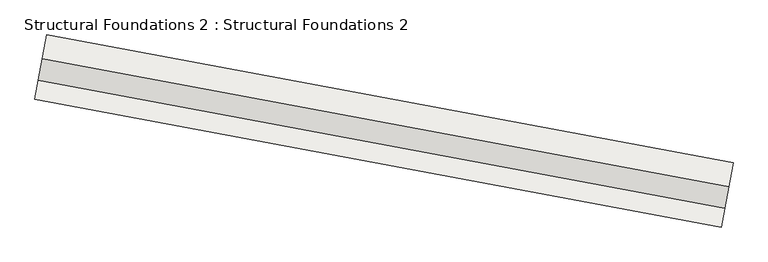
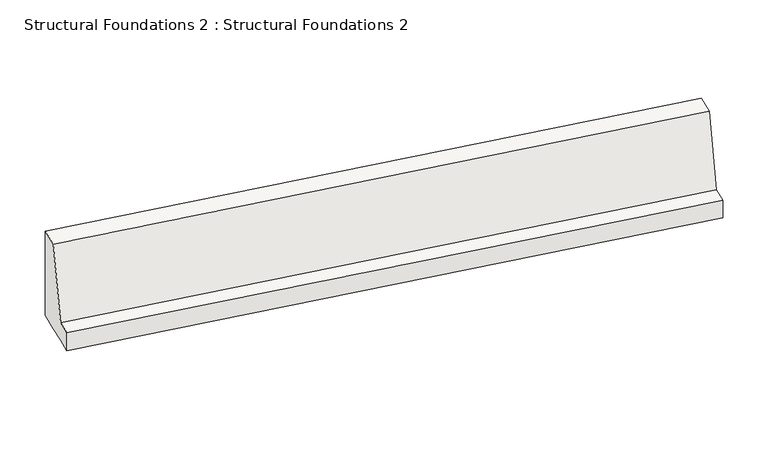
"""IFC4 building model written with IfcOpenShell, lengths in millimetres: slab geometry, Structural Foundations 2 : Structural Foundations 2."""

from ifc_helpers import new_model, si_unit, frame, origin, place, context, project, spatial, polyline, outline, extrude, source, transform, mapped, element, save


def structural_foundations_2_structural_foundations_2_d3b20905(model_context):
    return source(origin(), model_context, "Body", "SweptSolid", [
        extrude(outline(polyline([(0.0, 0.0), (0.0, -1930.4), (-457.2, -1930.4), (-863.6, -406.4), (-1219.2, -406.4), (-1219.2, 0.0), (-863.6, 0.0), (-457.2, 0.0), (0.0, 0.0)])), frame((-47568.5974532, 36188.2727948, 7848.6), z_axis=(-0.9830688624224049, 0.18323649127703542, 0.0), x_axis=(0.18323649127703542, 0.9830688624224049, 0.0)), (0.0, 0.0, 1.0), 13030.2),
    ])


if __name__ == "__main__":
    model = new_model("IFC4")
    model_context = context("Model", 3, world=origin())
    ifc_project = project(units=[si_unit("LENGTHUNIT", "METRE", prefix="MILLI")], contexts=[model_context])
    site = spatial("IfcSite", under=ifc_project)
    building = spatial("IfcBuilding", under=site)
    placement = place(None, origin())
    structural_foundations_2_structural_foundations_2_shape = structural_foundations_2_structural_foundations_2_d3b20905(model_context)
    element("IfcSlab", 1, ObjectType="Structural Foundations 2 : Structural Foundations 2", at=placement, inside=building, context=model_context, shape_type="MappedRepresentation", body=[
        mapped(structural_foundations_2_structural_foundations_2_shape, transform((0.0, 0.0, 0.0), x_axis=(1.0, 0.0, 0.0), y_axis=(0.0, 1.0, 0.0), z_axis=(0.0, 0.0, 1.0))),
    ])
    save(model, "model.ifc")

# Revit data of these elements
# Element 1 (IfcSlab, "Structural Foundations 2 : Structural Foundations 2")
#   Materials on its faces: "16 - Concrete - Cast-in-Place"
# Materials
#   "16 - Concrete - Cast-in-Place": class "Unassigned", colour RGB 192 192 192, transparency 0, Description = "Concrete", Cost = 0
